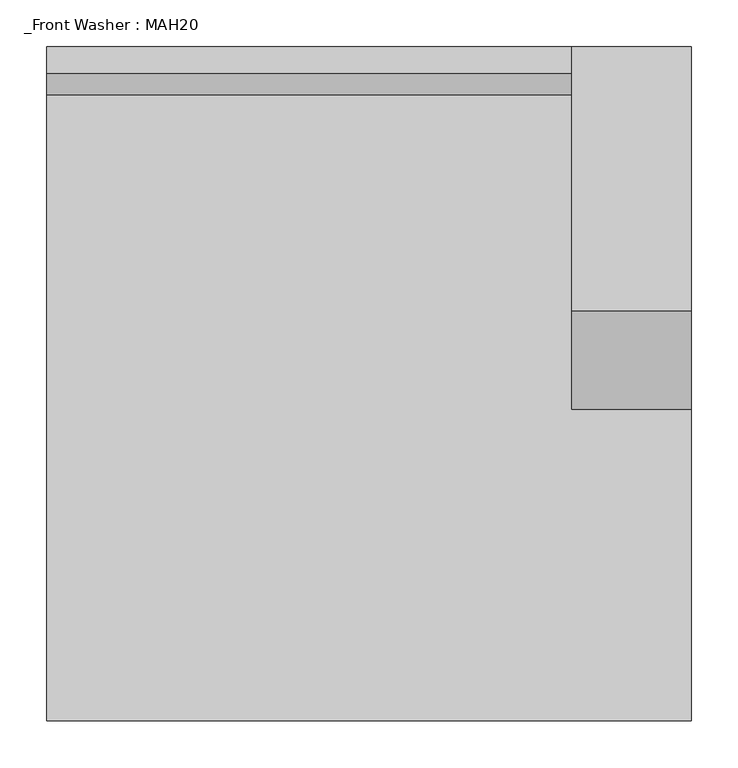
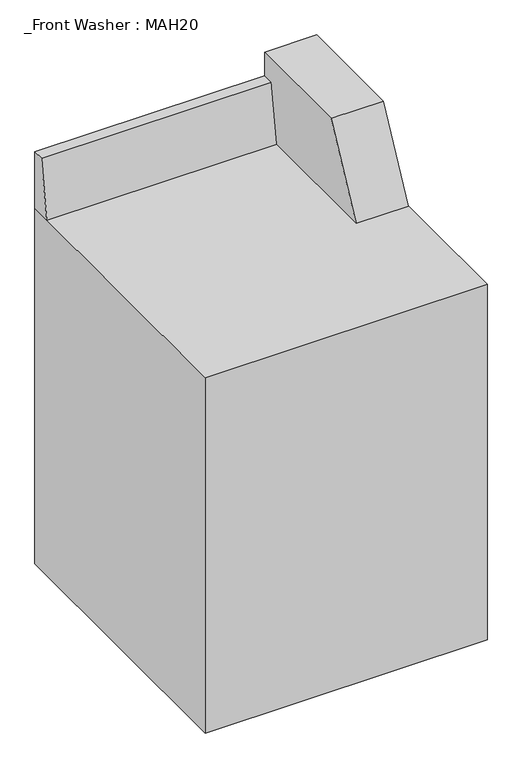
"""IFC4 building model written with IfcOpenShell, lengths in millimetres: proxy geometry, _Front Washer : MAH20."""

from ifc_helpers import new_model, si_unit, origin, origin_with_axes, place, context, project, spatial, polyline, outline, extrude, faceted_brep, source, transform, mapped, element, save


def front_washer_mah20_723598f1(model_context):
    return source(origin(), model_context, "Body", "SolidModel", [
        faceted_brep([(453.6513644, 717.55, 914.4), (453.6513644, 717.55, 1120.775), (453.6513644, 436.6694732, 1120.775), (453.6513644, 331.5520693, 914.4), (326.6513644, 331.5520693, 914.4), (326.6513644, 436.6694732, 1120.775), (326.6513644, 717.55, 1120.775), (326.6513644, 717.55, 1060.45), (326.6513644, 689.76875, 1060.45), (326.6513644, 666.75, 914.4), (-232.1486356, 666.75, 914.4), (-232.1486356, 717.55, 914.4), (-232.1486356, 717.55, 1060.45), (-232.1486356, 689.76875, 1060.45)], [[[0, 1, 2, 3]], [[4, 5, 6, 7, 8, 9]], [[2, 1, 6, 5]], [[3, 2, 5, 4]], [[3, 4, 9, 10, 11, 0]], [[6, 1, 0, 11, 12, 7]], [[12, 11, 10, 13]], [[12, 13, 8, 7]], [[13, 10, 9, 8]]]),
        extrude(outline(polyline([(453.6513644, 0.0), (-232.1486356, 0.0), (-232.1486356, 717.55), (453.6513644, 717.55), (453.6513644, 0.0)])), origin_with_axes(), (0.0, 0.0, 1.0), 914.4),
    ])


if __name__ == "__main__":
    model = new_model("IFC4")
    model_context = context("Model", 3, world=origin())
    ifc_project = project(units=[si_unit("LENGTHUNIT", "METRE", prefix="MILLI")], contexts=[model_context])
    site = spatial("IfcSite", under=ifc_project)
    building = spatial("IfcBuilding", under=site)
    placement = place(None, origin())
    front_washer_mah20_shape = front_washer_mah20_723598f1(model_context)
    element("IfcBuildingElementProxy", 1, Name="_Front Washer : MAH20", ObjectType="_Front Washer : MAH20", at=placement, inside=building, context=model_context, shape_type="MappedRepresentation", body=[
        mapped(front_washer_mah20_shape, transform((0.0, 0.0, 0.0), x_axis=(1.0, 0.0, 0.0), y_axis=(0.0, 1.0, 0.0), z_axis=(0.0, 0.0, 1.0))),
    ])
    save(model, "model.ifc")

# Revit data of these elements
# Type "_Front Washer : MAH20"
#   Type Mark = "MAH20"
#   Water_Pressure = "0"
#   Water_Flow_Rate = "0"
#   URL = "http://www.continentalgirbau.com"
#   Test Data = ""
#   Specification = "http://www.arcat.com/sd/clients/cogirbau.html?coid=44467"
#   SpecWizard = "http://www.arcat.com/specwizard/11110con/index.htm?mf=&coid=44467"
#   Send Message = "http://admin.arcat.com/users.pl?action=UserEmail&company=Continental%20Girbau,%20Inc.&coid=44467&rep=132&fax=920-231-4666 &mf="
#   Sales Information = ""
#   Product Properties = "http://www.arcat.com/bim/bim_info.pl?fn=Commercial_Washer"
#   Product Data = "http://www.arcat.com/arcatcos/cos44/arc44467.html"
#   Perf_WashSpeed = "44/67 rpm"
#   Perf_SpinSpeed = "710/473 rpm"
#   Perf_G-Force = "2.3/93 G"
#   Model = "H-Series"
#   Mech_Steam-Pressure = "29-87 psi"
#   Mech_Steam-Flow = "0"
#   Manufacturer Website = "http://www.continentalgirbau.com"
#   Manufacturer Phone - Toll Free = "800-256-1073 "
#   Manufacturer Phone = "920-231-8222 "
#   Manufacturer Fax = "920-231-4666 "
#   Manufacturer Address = "2500 State Rd. 44; Oshkosh; WI 54904\r\n"
#   Manufacturer = "Continental Girbau, Inc.\r\n"
#   Keynote = "11 23 00"
#   Installation-Fabrication = ""
#   Installation Phase = "Interior Fittings"
#   Green Building-LEED = "http://www.arcat.com/green/clients/leed_data_44467.html"
#   Drawn By = "Robert S. Weygant, CSI, CDT, SCIP"
#   Description = "Commercial Washer"
#   Copyright = "2009, ARCAT, Inc."
#   Construction Details = "http://www.arcat.com/details/cogirbau/cogirbau.html?coid=44467"
#   Compressed_Air_Pressure = "0"
#   Compressed_Air_Flow = "0"
#   Building Codes = ""
#   Assembly Code = "E1010610"
#   Three Phase = 0 VA
#   Single Phase = 0 VA
#   VOLTAGE = 120 V
#   OpeningCL = 0' - 7 7/8"
#   Mech_steam = 0' - 0 1/2"
#   Mech_HW = 0' - 0 3/8"
#   Mech_CW = 0' - 0 3/8"
#   MechWaste = 0' - 0 3/8"
#   MachWidth = 2' - 3"
#   MachHeight = 3' - 0"
#   MachDepth = 2' - 4 1/4"
#   LwrPanHt = 1' - 0"
#   InstWidth = 1' - 7 69/256"
#   Height of Back Panel = 3' - 5 3/4"
#   Height at Coin Insert = 3' - 8 1/8"
#   GlassCL = 0' - 5 7/8"
#   Fr_FaceWdth = 0' - 4 1/2"
#   DoorOpening = 1' - 3 3/4"
#   DoorHeight = 1' - 6"
#   Cyl_Diam = 1' - 0"
#   Cyl_Depth = 1' - 9"
#   CylRad = 0' - 6"
#   Compressed_Air_Connection = 0' - 2"
#   Capacity_Weight = 55
#   Capacity_Volume = 1.37445 (stored number, unit not read)
#   Warranty Duration (Years) = 0
#   Maintenance Schedule (Months) = 0
#   Expected Lifespan (Years) = 0
#   Trim Material = Painted Metal - Black
#   Shell Material = Stainless Steel
# Element 1 (IfcBuildingElementProxy, "_Front Washer : MAH20")
#   Materials on its faces: "Stainless Steel"
# Materials
#   "Painted Metal - Black": class "Unassigned", colour RGB 223 223 223, transparency 0, Cost = 0
#   "Stainless Steel": class "Unassigned", colour RGB 247 247 247, transparency 0
